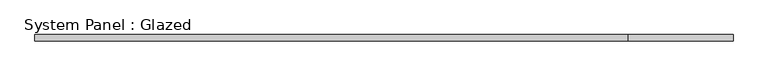
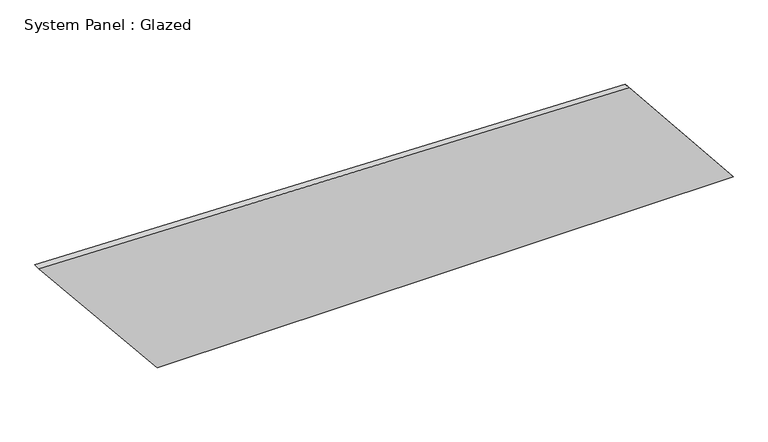
"""IFC4 building model written with IfcOpenShell, lengths in millimetres: plate geometry, System Panel : Glazed."""

from ifc_helpers import new_model, si_unit, frame, origin, place, context, project, spatial, polyline, outline, extrude, source, transform, mapped, element, save


def system_panel_glazed_e32ca1c0(model_context):
    return source(origin(), model_context, "Body", "SweptSolid", [
        extrude(outline(polyline([(0.0, -896.5162129), (0.0, 1361.8416027), (511.6831474, 953.7486852), (573.6206829, -1361.8416027), (0.0, -896.5162129)])), frame((0.0, -49.5, 0.0), z_axis=(0.0, 1.0, 0.0), x_axis=(0.0, 0.0, 1.0)), (0.0, 0.0, 1.0), 25.0),
    ])


if __name__ == "__main__":
    model = new_model("IFC4")
    model_context = context("Model", 3, world=origin())
    ifc_project = project(units=[si_unit("LENGTHUNIT", "METRE", prefix="MILLI")], contexts=[model_context])
    site = spatial("IfcSite", under=ifc_project)
    building = spatial("IfcBuilding", under=site)
    placement = place(None, origin())
    system_panel_glazed_shape = system_panel_glazed_e32ca1c0(model_context)
    element("IfcPlate", 1, ObjectType="System Panel : Glazed", at=placement, inside=building, context=model_context, shape_type="MappedRepresentation", body=[
        mapped(system_panel_glazed_shape, transform((0.0, 0.0, 0.0), x_axis=(1.0, 0.0, 0.0), y_axis=(0.0, 1.0, 0.0), z_axis=(0.0, 0.0, 1.0))),
    ])
    save(model, "model.ifc")

# Revit data of these elements
# Element 1 (IfcPlate, "System Panel : Glazed")
#   Materials on its faces: "Glass, Clear Glazing"
# Materials
#   "Glass, Clear Glazing": class "Glass", colour RGB 247 249 248, transparency 0.85, Description = "Clear glazing", Cost = 0
